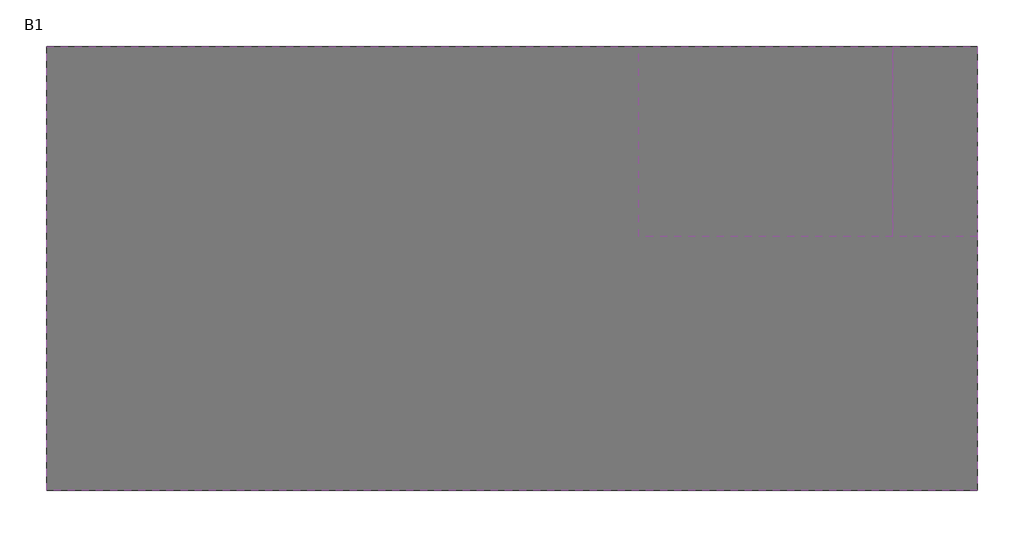
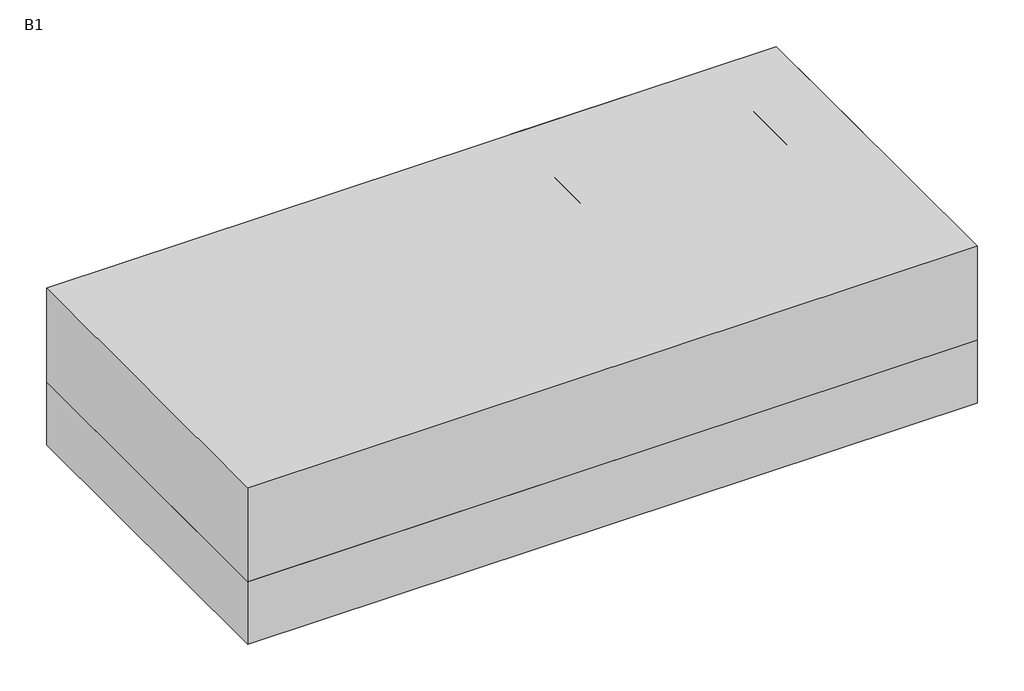
# One storey: 5 proxies.
"""IFC4 building model written with IfcOpenShell, lengths in millimetres."""

import ifcopenshell
import ifcopenshell.guid

model = None  # the IFC model being written
_history = None  # IfcOwnerHistory: only IFC2X3 demands one
_inside = {}  # id of a spatial element -> (the spatial element, [elements in it])
_under = {}  # id of a project, library or spatial element -> (it, [spatial elements below it])
_declared = {}  # id of a project -> (the project, [libraries it declares])
_typed = {}  # id of a type object -> (the type object, [elements of that type])
_made_of = {}  # id of a material, layer set ... -> (it, [elements and type objects made of it])


def new_model(schema):
    """Start an empty IFC model of exactly this schema.

    Asked for "IFC4X3", IfcOpenShell would pick the latest addendum, in which some entities
    have other attributes; the version numbers below select the first issue.
    IFC2X3 requires an IfcOwnerHistory on every rooted entity: one is made here for all.
    """
    global model, _history
    if schema == "IFC4X3":
        model = ifcopenshell.file(schema_version=(4, 3, 0, 0))
    else:
        model = ifcopenshell.file(schema=schema)
    _inside.clear()
    _under.clear()
    _declared.clear()
    _typed.clear()
    _made_of.clear()
    _history = None
    if model.schema == "IFC2X3":
        org = make("IfcOrganization", Name="unknown")
        user = make(
            "IfcPersonAndOrganization",
            ThePerson=make("IfcPerson", FamilyName="unknown"),
            TheOrganization=org,
        )
        app = make(
            "IfcApplication",
            ApplicationDeveloper=org,
            Version="unknown",
            ApplicationFullName="unknown",
            ApplicationIdentifier="unknown",
        )
        _history = make(
            "IfcOwnerHistory",
            OwningUser=user,
            OwningApplication=app,
            ChangeAction="ADDED",
            CreationDate=0,
        )
    return model


def make(cls, **values):
    """One entity of the class cls with the attributes given. An attribute that is None is left unset."""
    return model.create_entity(
        cls, **{name: value for name, value in values.items() if value is not None}
    )


def rooted(cls, **values):
    """An entity with a GlobalId (a new one), such as an element, a storey or a relation."""
    return make(cls, GlobalId=ifcopenshell.guid.new(), OwnerHistory=_history, **values)


def si_unit(unit_type, name, prefix=None):
    """IfcSIUnit, for example si_unit("LENGTHUNIT", "METRE", prefix="MILLI")."""
    return make("IfcSIUnit", UnitType=unit_type, Prefix=prefix, Name=name)


def assignment(units):
    """IfcUnitAssignment: the units of a project."""
    return None if units is None else make("IfcUnitAssignment", Units=units)


def point(xyz):
    """IfcCartesianPoint."""
    return None if xyz is None else make("IfcCartesianPoint", Coordinates=xyz)


def direction(xyz):
    """IfcDirection."""
    return None if xyz is None else make("IfcDirection", DirectionRatios=xyz)


def frame(location, z_axis=None, x_axis=None):
    """IfcAxis2Placement3D, a coordinate frame: its origin and axes. An axis left out is left unset."""
    return make(
        "IfcAxis2Placement3D",
        Location=point(location),
        Axis=direction(z_axis),
        RefDirection=direction(x_axis),
    )


def origin():
    """The frame at (0, 0, 0) with its axes left unset."""
    return frame((0.0, 0.0, 0.0))


def origin_with_axes():
    """The frame at (0, 0, 0) with the z axis (0, 0, 1) and the x axis (1, 0, 0) written out."""
    return frame((0.0, 0.0, 0.0), z_axis=(0.0, 0.0, 1.0), x_axis=(1.0, 0.0, 0.0))


def place(relative_to, where):
    """IfcLocalPlacement: puts the frame where relative to a parent placement (None: the world)."""
    return make(
        "IfcLocalPlacement", PlacementRelTo=relative_to, RelativePlacement=where
    )


def context(
    kind, dimensions, precision=None, world=None, true_north=None, identifier=None
):
    """IfcGeometricRepresentationContext, for example the 3D "Model" context."""
    return make(
        "IfcGeometricRepresentationContext",
        ContextIdentifier=identifier,
        ContextType=kind,
        CoordinateSpaceDimension=dimensions,
        Precision=precision,
        WorldCoordinateSystem=world,
        TrueNorth=true_north,
    )


def project(units=None, contexts=None):
    """IfcProject with its units and contexts."""
    return rooted(
        "IfcProject",
        Name="project",
        RepresentationContexts=contexts,
        UnitsInContext=assignment(units),
    )


def spatial(cls, under=None, at=None, **own):
    """A site, building, storey or space (cls), placed at a placement, below another one or the project."""
    s = rooted(cls, ObjectPlacement=at, **own)
    if under is not None:
        _under.setdefault(under.id(), (under, []))[1].append(s)
    return s


def polyline(points):
    """IfcPolyline through the points."""
    return make("IfcPolyline", Points=[point(p) for p in points])


def outline(outer, holes=None, kind="AREA"):
    """IfcArbitraryClosedProfileDef: a profile drawn as a closed curve; with holes, ...WithVoids."""
    if holes is None:
        return make("IfcArbitraryClosedProfileDef", ProfileType=kind, OuterCurve=outer)
    return make(
        "IfcArbitraryProfileDefWithVoids",
        ProfileType=kind,
        OuterCurve=outer,
        InnerCurves=holes,
    )


def extrude(swept, where, along, depth):
    """IfcExtrudedAreaSolid: the profile swept, set in the frame where, extruded along a direction by depth."""
    return make(
        "IfcExtrudedAreaSolid",
        SweptArea=swept,
        Position=where,
        ExtrudedDirection=direction(along),
        Depth=depth,
    )


def shape(context_of_items, identifier, shape_type, items):
    """IfcShapeRepresentation: the items that make up one representation, for example the "Body"."""
    return make(
        "IfcShapeRepresentation",
        ContextOfItems=context_of_items,
        RepresentationIdentifier=identifier,
        RepresentationType=shape_type,
        Items=items,
    )


def source(mapping_origin, context_of_items, identifier, shape_type, items):
    """IfcRepresentationMap: a shape defined once, which mapped items show again and again."""
    return make(
        "IfcRepresentationMap",
        MappingOrigin=mapping_origin,
        MappedRepresentation=shape(context_of_items, identifier, shape_type, items),
    )


def transform(
    local_origin,
    x_axis=None,
    y_axis=None,
    z_axis=None,
    scale=None,
    scale2=None,
    scale3=None,
    uniform=True,
):
    """IfcCartesianTransformationOperator3D, or its non-uniform kind. x_axis, y_axis, z_axis: its Axis1, 2, 3."""
    if uniform:
        return make(
            "IfcCartesianTransformationOperator3D",
            Axis1=direction(x_axis),
            Axis2=direction(y_axis),
            LocalOrigin=point(local_origin),
            Scale=scale,
            Axis3=direction(z_axis),
        )
    return make(
        "IfcCartesianTransformationOperator3DnonUniform",
        Axis1=direction(x_axis),
        Axis2=direction(y_axis),
        LocalOrigin=point(local_origin),
        Scale=scale,
        Axis3=direction(z_axis),
        Scale2=scale2,
        Scale3=scale3,
    )


def mapped(mapping_source, mapping_target):
    """IfcMappedItem: shows the shape of a source again, moved by a transform."""
    return make(
        "IfcMappedItem", MappingSource=mapping_source, MappingTarget=mapping_target
    )


def made_of(thing, what):
    """Note that an element or type object is made of a material, layer set ...; save() writes the relation."""
    if what is not None:
        _made_of.setdefault(what.id(), (what, []))[1].append(thing)
    return thing


def element(
    cls,
    number,
    at=None,
    inside=None,
    cuts=None,
    type_object=None,
    material=None,
    context=None,
    identifier="Body",
    shape_type=None,
    held_by="IfcProductDefinitionShape",
    body=None,
    shapes=None,
    **own,
):
    """One element of the class cls, such as IfcWall. Its Tag is "e" and its number.

    at: its placement. inside: the storey or other place that contains it. cuts: it is an
    opening in that element (IfcRelVoidsElement). A single representation is given by context,
    identifier, shape_type and body (its items); several are given by shapes. held_by: the class
    of the entity that holds the representations. save() writes the other relations.
    """
    e = rooted(cls, Tag="e%d" % number, ObjectPlacement=at, **own)
    if body is not None:
        shapes = [shape(context, identifier, shape_type, body)]
    if shapes is not None:
        e.Representation = make(held_by, Representations=shapes)
    if inside is not None:
        _inside.setdefault(inside.id(), (inside, []))[1].append(e)
    if cuts is not None:
        rooted(
            "IfcRelVoidsElement", RelatingBuildingElement=cuts, RelatedOpeningElement=e
        )
    if type_object is not None:
        _typed.setdefault(type_object.id(), (type_object, []))[1].append(e)
    return made_of(e, material)


def aggregate(whole, parts):
    """IfcRelAggregates: a whole, such as a stair, and the parts it consists of."""
    return rooted("IfcRelAggregates", RelatingObject=whole, RelatedObjects=parts)


def save(model, path):
    """Write the relations noted so far, then the file.

    IfcRelAggregates (storeys below a building ...), IfcRelContainedInSpatialStructure (elements
    in a storey), IfcRelDefinesByType, IfcRelAssociatesMaterial and IfcRelDeclares: one each for
    every whole, place, type object, material and project.
    """
    for whole, parts in _under.values():
        aggregate(whole, parts)
    for where, things in _inside.values():
        rooted(
            "IfcRelContainedInSpatialStructure",
            RelatedElements=things,
            RelatingStructure=where,
        )
    for kind, things in _typed.values():
        rooted("IfcRelDefinesByType", RelatedObjects=things, RelatingType=kind)
    for what, things in _made_of.values():
        rooted("IfcRelAssociatesMaterial", RelatedObjects=things, RelatingMaterial=what)
    for by, libraries in _declared.values():
        rooted("IfcRelDeclares", RelatingContext=by, RelatedDefinitions=libraries)
    model.write(path)


def generic_models_399a6151(model_context):
    return source(origin(), model_context, "Body", "SweptSolid", [
        extrude(outline(polyline([(4500.0, 6000.0), (4500.0, -6000.0), (-4500.0, -6000.0), (-4500.0, 6000.0), (4500.0, 6000.0)])), origin_with_axes(), (0.0, 0.0, 1.0), 6000.0),
    ])


def generic_models_29bcd6f9(model_context):
    return source(origin(), model_context, "Body", "SweptSolid", [
        extrude(outline(polyline([(2000.0, 4500.0), (2000.0, -4500.0), (-2000.0, -4500.0), (-2000.0, 4500.0), (2000.0, 4500.0)])), origin_with_axes(), (0.0, 0.0, 1.0), 6000.0),
    ])


def generic_models_a454a2aa(model_context):
    return source(origin(), model_context, "Body", "SweptSolid", [
        extrude(outline(polyline([(10500.0, 22000.0), (10500.0, -22000.0), (-10500.0, -22000.0), (-10500.0, 22000.0), (10500.0, 22000.0)])), origin_with_axes(), (0.0, 0.0, 1.0), 4000.0),
    ])


def generic_models_73802227(model_context):
    return source(origin(), model_context, "Body", "SweptSolid", [
        extrude(outline(polyline([(2000.0, 4500.0), (2000.0, -4500.0), (-2000.0, -4500.0), (-2000.0, 4500.0), (2000.0, 4500.0)])), origin_with_axes(), (0.0, 0.0, 1.0), 4000.0),
    ])


def generic_models_7e8091d6(model_context):
    return source(origin(), model_context, "Body", "SweptSolid", [
        extrude(outline(polyline([(22000.0, 10500.0), (22000.0, -10500.0), (-22000.0, -10500.0), (-22000.0, 10500.0), (22000.0, 10500.0)])), origin_with_axes(), (0.0, 0.0, 1.0), 6000.0),
    ])


model = new_model("IFC4")

# Units and contexts
model_context = context("Model", 3, world=origin())
ifc_project = project(units=[si_unit("LENGTHUNIT", "METRE", prefix="MILLI")], contexts=[model_context])

# Site, building, storey
site = spatial("IfcSite", under=ifc_project)
building = spatial("IfcBuilding", under=site)
storey = spatial("IfcBuildingStorey", under=building, Name="B1", Elevation=-4000.0)

# Proxies
placement = place(None, origin())
generic_models_shape = generic_models_399a6151(model_context)
element("IfcBuildingElementProxy", 1, Name="Space Planning Box_hec : Space Planning Box_hec", ObjectType="Space Planning Box_hec : Space Planning Box_hec", at=placement, inside=storey, context=model_context, shape_type="MappedRepresentation", body=[
    mapped(generic_models_shape, transform((79459.6521483, 180423.8614395, 0.0), x_axis=(0.0, -1.0, 0.0), y_axis=(1.0, 0.0, 0.0), z_axis=(0.0, 0.0, 1.0))),
])
generic_models_2_shape = generic_models_29bcd6f9(model_context)
element("IfcBuildingElementProxy", 2, Name="Space Planning Box_hec : Space Planning Box_hec", ObjectType="Space Planning Box_hec : Space Planning Box_hec", at=placement, inside=storey, context=model_context, shape_type="MappedRepresentation", body=[
    mapped(generic_models_2_shape, transform((87459.6521483, 180423.8614395, 0.0), x_axis=(1.0, 0.0, 0.0), y_axis=(0.0, 1.0, 0.0), z_axis=(0.0, 0.0, 1.0))),
])
generic_models_3_shape = generic_models_a454a2aa(model_context)
element("IfcBuildingElementProxy", 3, Name="Space Planning Box_hec : Space Planning Box_hec", ObjectType="Space Planning Box_hec : Space Planning Box_hec", at=placement, inside=storey, context=model_context, shape_type="MappedRepresentation", body=[
    mapped(generic_models_3_shape, transform((67459.6521483, 174423.8614395, -4000.0), x_axis=(0.0, -1.0, 0.0), y_axis=(1.0, 0.0, 0.0), z_axis=(0.0, 0.0, 1.0))),
])
generic_models_4_shape = generic_models_73802227(model_context)
element("IfcBuildingElementProxy", 4, Name="Space Planning Box_hec : Space Planning Box_hec", ObjectType="Space Planning Box_hec : Space Planning Box_hec", at=placement, inside=storey, context=model_context, shape_type="MappedRepresentation", body=[
    mapped(generic_models_4_shape, transform((87459.6521483, 180423.8614395, -4000.0), x_axis=(1.0, 0.0, 0.0), y_axis=(0.0, 1.0, 0.0), z_axis=(0.0, 0.0, 1.0))),
])
generic_models_5_shape = generic_models_7e8091d6(model_context)
element("IfcBuildingElementProxy", 5, Name="Space Planning Box_hec : Space Planning Box_hec", ObjectType="Space Planning Box_hec : Space Planning Box_hec", at=placement, inside=storey, context=model_context, shape_type="MappedRepresentation", body=[
    mapped(generic_models_5_shape, transform((67459.6521483, 174423.8614395, 0.0), x_axis=(1.0, 0.0, 0.0), y_axis=(0.0, 1.0, 0.0), z_axis=(0.0, 0.0, 1.0))),
])

save(model, "model.ifc")

# Revit data of these elements
# Project information
#   Building Name = "MAIN GATE SECURITY BUILDING"
#   Project Status = "Project Status"
#   Client Name = "현대엔지니어링"
#   Project Address = "서울시 종로구 율곡로 75(계동)"
#   Project Name = "Therma Visayas Energy Project"
#   Project Number = "-"
# Grids (mm)
#   "A": line (45459.652, 190234.526) -> (45459.652, 152139.384)
#   "B": line (53459.652, 190234.526) -> (53459.652, 152139.384)
#   "C": line (61459.652, 190234.526) -> (61459.652, 152139.384)
#   "D": line (67459.652, 190234.526) -> (67459.652, 152139.384)
#   "E": line (73459.652, 190234.526) -> (73459.652, 152139.384)
#   "F": line (81459.652, 190234.526) -> (81459.652, 152139.384)
#   "G": line (85459.652, 190234.526) -> (85459.652, 152139.384)
#   "H": line (89459.652, 190234.526) -> (89459.652, 152139.384)
#   "4": line (39389.066, 184923.861) -> (102402.798, 184923.861)
#   "3": line (39389.066, 178923.861) -> (102402.798, 178923.861)
#   "2": line (39389.066, 172923.861) -> (102402.798, 172923.861)
#   "1": line (39389.066, 163923.861) -> (102402.798, 163923.861)
# Type "Space Planning Box_hec : Space Planning Box_hec"
#   Type Comments = "..."
#   Room Name [instance default] = "?"
#   Interior Finish [instance default] = ""
#   Exterior Finish [instance default] = ""
#   Department [instance default] = ""
#   Assembly Code = "..."
#   Width [instance default] = 1524 mm
#   Program Area [instance default] = 0.00 m²
#   Length [instance default] = 1524 mm
#   Height [instance default] = 1524 mm
#   Area [instance default] = 2.32258 m²
#   Fill Color [instance default] = Cyan
#   Default Elevation = 0
# Element 1 (IfcBuildingElementProxy, "Space Planning Box_hec : Space Planning Box_hec")
#   Room Name = "Battery Room"
#   Interior Finish = "IF4"
#   Exterior Finish = "EF1"
#   Department = "EL"
#   Width = 9000 mm
#   Program Area = 108.00 m²
#   Length = 12000 mm
#   Height = 6000 mm
#   Area = 108.00 m²
#   Fill Color = Blue
#   Phase Created = New Construction
#   Materials on its faces: "Blue"
# Element 2 (IfcBuildingElementProxy, "Space Planning Box_hec : Space Planning Box_hec")
#   Room Name = "Stairway"
#   Interior Finish = "IF2"
#   Exterior Finish = "EF1"
#   Department = "AR"
#   Width = 4000 mm
#   Program Area = 36.00 m²
#   Length = 9000 mm
#   Height = 6000 mm
#   Area = 36.00 m²
#   Fill Color = Lavender
#   Phase Created = New Construction
#   Materials on its faces: "Lavender"
# Element 3 (IfcBuildingElementProxy, "Space Planning Box_hec : Space Planning Box_hec")
#   Room Name = "Cable Room"
#   Interior Finish = "IF1"
#   Exterior Finish = "EF1"
#   Department = "EL"
#   Width = 21000 mm
#   Program Area = 924.00 m²
#   Length = 44000 mm
#   Height = 4000 mm
#   Area = 924.00 m²
#   Fill Color = Blue
#   Phase Created = New Construction
#   Materials on its faces: "Blue"
# Element 4 (IfcBuildingElementProxy, "Space Planning Box_hec : Space Planning Box_hec")
#   Room Name = "Stairway"
#   Interior Finish = "IF2"
#   Exterior Finish = "EF1"
#   Department = "AR"
#   Width = 4000 mm
#   Program Area = 36.00 m²
#   Length = 9000 mm
#   Height = 4000 mm
#   Area = 36.00 m²
#   Fill Color = Lavender
#   Phase Created = New Construction
#   Materials on its faces: "Lavender"
# Element 5 (IfcBuildingElementProxy, "Space Planning Box_hec : Space Planning Box_hec")
#   Room Name = "Switchgear Room"
#   Interior Finish = "IF1"
#   Exterior Finish = "EF1"
#   Department = "EL"
#   Width = 44000 mm
#   Program Area = 58.50 m²
#   Length = 21000 mm
#   Height = 6000 mm
#   Area = 924.00 m²
#   Fill Color = Blue
#   Phase Created = New Construction
#   Materials on its faces: "Blue"
# Materials
#   "Cyan": class "Generic", colour RGB 0 255 255, transparency 0.2, Cost = 0
#   "Blue": class "Generic", colour RGB 0 0 255, transparency 0.2, Cost = 0
#   "Lavender": class "Generic", colour RGB 186 85 211, transparency 0.2, Cost = 0
